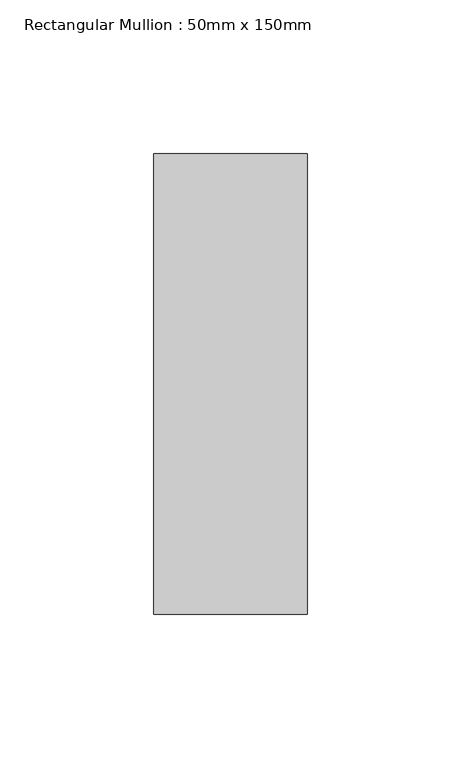
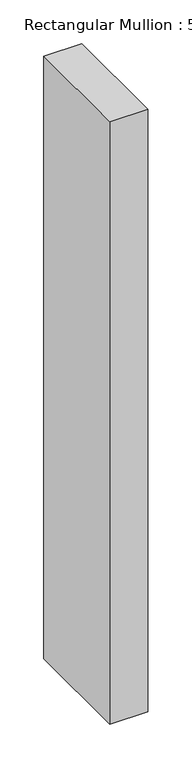
"""IFC4 building model written with IfcOpenShell, lengths in millimetres: member geometry, Rectangular Mullion : 50mm x 150mm."""

from ifc_helpers import new_model, si_unit, frame, origin, place, context, project, spatial, polyline, outline, extrude, source, transform, mapped, element, save


def rectangular_mullion_50mm_x_150mm_2b7f9caa(model_context):
    return source(origin(), model_context, "Body", "SweptSolid", [
        extrude(outline(polyline([(0.0, 75.0), (0.0, -75.0), (-50.0, -75.0), (-50.0, 75.0), (0.0, 75.0)])), frame((0.0, 0.0, -837.8787879), z_axis=(0.0, 0.0, 1.0), x_axis=(1.0, 0.0, 0.0)), (0.0, 0.0, 1.0), 837.8787879),
    ])


if __name__ == "__main__":
    model = new_model("IFC4")
    model_context = context("Model", 3, world=origin())
    ifc_project = project(units=[si_unit("LENGTHUNIT", "METRE", prefix="MILLI")], contexts=[model_context])
    site = spatial("IfcSite", under=ifc_project)
    building = spatial("IfcBuilding", under=site)
    placement = place(None, origin())
    rectangular_mullion_50mm_x_150mm_shape = rectangular_mullion_50mm_x_150mm_2b7f9caa(model_context)
    element("IfcMember", 1, ObjectType="Rectangular Mullion : 50mm x 150mm", at=placement, inside=building, context=model_context, shape_type="MappedRepresentation", body=[
        mapped(rectangular_mullion_50mm_x_150mm_shape, transform((0.0, 0.0, 0.0), x_axis=(1.0, 0.0, 0.0), y_axis=(0.0, 1.0, 0.0), z_axis=(0.0, 0.0, 1.0))),
    ])
    save(model, "model.ifc")

# Revit data of these elements
# Type "Rectangular Mullion : 50mm x 150mm"
#   built-in parameter 1007304 = 0.492126 (stored number, unit not read)
#   built-in parameter 1007301 = 0.082021 (stored number, unit not read)
#   built-in parameter 1007300 = 0.082021 (stored number, unit not read)
# Element 1 (IfcMember, "Rectangular Mullion : 50mm x 150mm")
#   Materials on its faces: "Aluminum"
# Materials
#   "Aluminum": class "Metal", colour RGB 244 244 244, transparency 0, Description = "Aluminum 6061", Cost = 0
